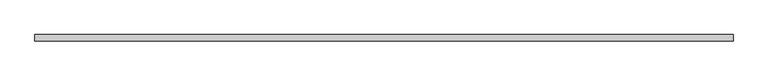
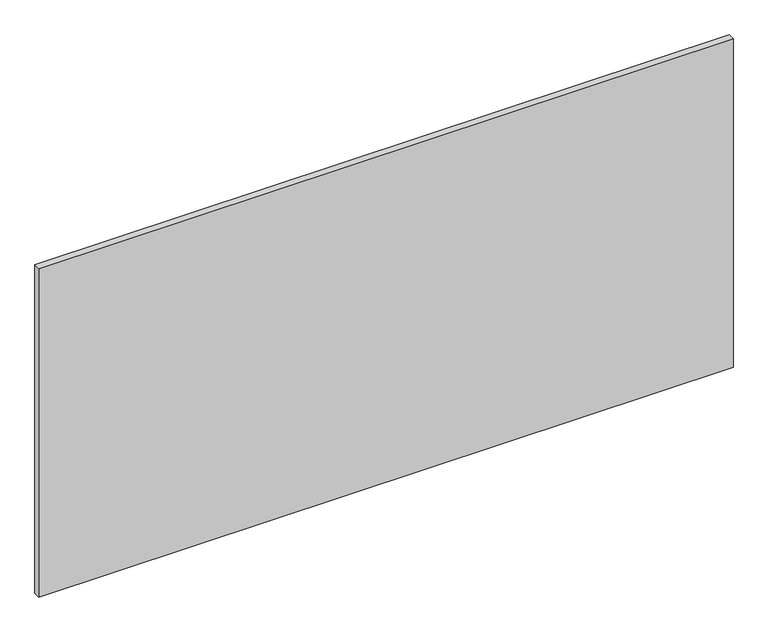
"""IFC4 building model written with IfcOpenShell, lengths in millimetres: proxy geometry, Inner panel:Inner panel:1:Inner panel:1 : Inner panel:Inner panel:300324:300043:Inner panel:1:Inner panel:1 : Inner panel:Inner panel:300324:300043 : Inner panel:Inner panel:1:Inner panel:1 : Inner panel:Inner panel:300324:300043:7 : Inner panel:Inner panel:1:Inner panel:1 : Inner panel:Inner panel:300324:300043:Inner panel:1:Inner panel:1 : Inner panel:Inner panel:300324:300043 : Inner panel:Inner panel:1:Inner panel:1 : Inner panel:Inner panel:300324:300043:300031."""

from ifc_helpers import new_model, si_unit, frame, origin, place, context, project, spatial, polyline, outline, extrude, source, transform, mapped, element, save


def generic_models_d0613c39(model_context):
    return source(origin(), model_context, "Body", "SweptSolid", [
        extrude(outline(polyline([(570452.6367239, -579000.6913841), (572891.0367239, -579000.6913841), (572891.0367239, -579022.9163841), (570452.6367239, -579022.9163841), (570452.6367239, -579000.6913841)])), frame((0.0, 0.0, 1270.0), z_axis=(0.0, 0.0, 1.0), x_axis=(1.0, 0.0, 0.0)), (0.0, 0.0, 1.0), 1219.2),
    ])


if __name__ == "__main__":
    model = new_model("IFC4")
    model_context = context("Model", 3, world=origin())
    ifc_project = project(units=[si_unit("LENGTHUNIT", "METRE", prefix="MILLI")], contexts=[model_context])
    site = spatial("IfcSite", under=ifc_project)
    building = spatial("IfcBuilding", under=site)
    placement = place(None, origin())
    generic_models_shape = generic_models_d0613c39(model_context)
    element("IfcBuildingElementProxy", 1, Name="Inner panel:Inner panel:1:Inner panel:1 : Inner panel:Inner panel:300324:300043:Inner panel:1:Inner panel:1 : Inner panel:Inner panel:300324:300043 : Inner panel:Inner panel:1:Inner panel:1 : Inner panel:Inner panel:300324:300043:7 : Inner panel:Inner panel:1:Inner panel:1 : Inner panel:Inner panel:300324:300043:Inner panel:1:Inner panel:1 : Inner panel:Inner panel:300324:300043 : Inner panel:Inner panel:1:Inner panel:1 : Inner panel:Inner panel:300324:300043:300031", ObjectType="Inner panel:Inner panel:1:Inner panel:1 : Inner panel:Inner panel:300324:300043:Inner panel:1:Inner panel:1 : Inner panel:Inner panel:300324:300043 : Inner panel:Inner panel:1:Inner panel:1 : Inner panel:Inner panel:300324:300043:7 : Inner panel:Inner panel:1:Inner panel:1 : Inner panel:Inner panel:300324:300043:Inner panel:1:Inner panel:1 : Inner panel:Inner panel:300324:300043 : Inner panel:Inner panel:1:Inner panel:1 : Inner panel:Inner panel:300324:300043:300031", at=placement, inside=building, context=model_context, shape_type="MappedRepresentation", body=[
        mapped(generic_models_shape, transform((0.0, 0.0, 0.0), x_axis=(1.0, 0.0, 0.0), y_axis=(0.0, 1.0, 0.0), z_axis=(0.0, 0.0, 1.0))),
    ])
    save(model, "model.ifc")

# Revit data of these elements
# Type "Inner panel:Inner panel:1:Inner panel:1 : Inner panel:Inner panel:300324:300043:Inner panel:1:Inner panel:1 : Inner panel:Inner panel:300324:300043 : Inner panel:Inner panel:1:Inner panel:1 : Inner panel:Inner panel:300324:300043:7 : Inner panel:Inner panel:1:Inner panel:1 : Inner panel:Inner panel:300324:300043:Inner panel:1:Inner panel:1 : Inner panel:Inner panel:300324:300043 : Inner panel:Inner panel:1:Inner panel:1 : Inner panel:Inner panel:300324:300043:300031"
#   NameOverride = "Inner panel:Inner panel:1:Inner panel:1 : Inner panel:Inner panel:300324:300043:Inner panel:1:Inner panel:1 : Inner panel:Inner panel:300324:300043 : Inner panel:Inner panel:1:Inner panel:1 : Inner panel:Inner panel:300324:300043:300031"
#   ObjectTypeOverride = "Inner panel:1:Inner panel:1 : Inner panel:Inner panel:300324:300043 : Inner panel:Inner panel:1:Inner panel:1 : Inner panel:Inner panel:300324:300043"
#   Reference = "Inner panel"
#   Tag = "300031"
# Element 1 (IfcBuildingElementProxy, "Inner panel:Inner panel:1:Inner panel:1 : Inner panel:Inner panel:300324:300043:Inner panel:1:Inner panel:1 : Inner panel:Inner panel:300324:300043 : Inner panel:Inner panel:1:Inner panel:1 : Inner panel:Inner panel:300324:300043:7 : Inner panel:Inner panel:1:Inner panel:1 : Inner panel:Inner panel:300324:300043:Inner panel:1:Inner panel:1 : Inner panel:Inner panel:300324:300043 : Inner panel:Inner panel:1:Inner panel:1 : Inner panel:Inner panel:300324:300043:300031")
#   Materials on its faces: "1/2\" EXTERIOR GRADE FIRE RETARDANT CDX PLYWOOD"
# Materials
#   "1/2\" EXTERIOR GRADE FIRE RETARDANT CDX PLYWOOD": class "Unassigned", colour RGB 196 177 123, transparency 0, Cost = 0
